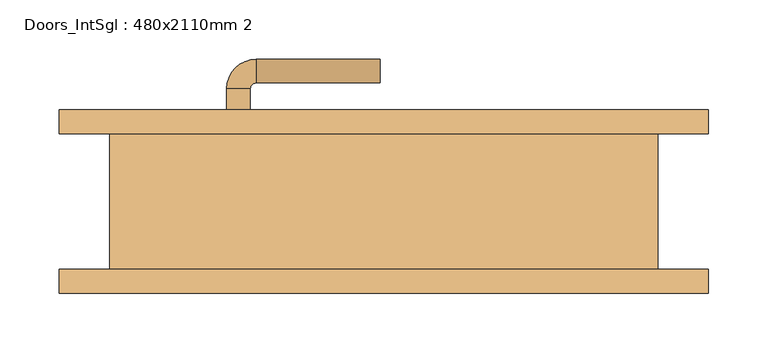
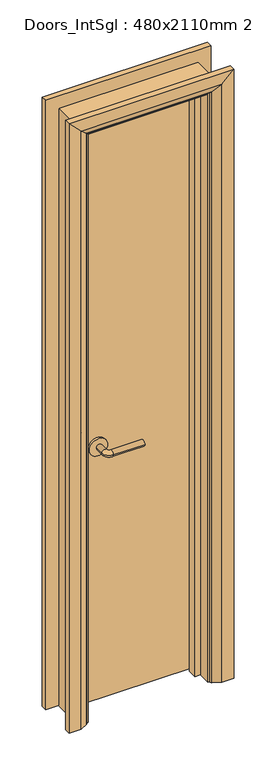
"""IFC4 building model written with IfcOpenShell, lengths in millimetres: door geometry, Doors_IntSgl : 480x2110mm 2."""

from ifc_helpers import new_model, si_unit, point, frame, frame_2d, origin, place, context, project, spatial, polyline, circle_curve, ellipse_curve, trimmed, segment, composite_curve, outline, extrude, faceted_brep, source, transform, mapped, element, save
from ifc_brep_helpers import plane_surface, cylinder_surface, revolved_surface, advanced_brep


def doors_intsgl_480x2110mm_2_fe7a8983(model_context):
    return source(origin(), model_context, "Body", "SolidModel", [
        advanced_brep(
        [(-133.0, 11.5, 900.0), (-113.0, 11.5, 900.0), (-113.0, -18.5, 900.0), (-133.0, -18.5, 900.0), (-108.0, -23.5, 900.0), (-108.0, -43.5, 900.0), (-3.0, -43.5, 900.0), (-3.0, -23.5, 900.0)],
        [
            (0, 1, circle_curve(frame((-123.0, 11.5, 900.0), z_axis=(0.0, 1.0, 0.0), x_axis=(1.0, 0.0, 0.0)), 10.0)),
            (1, 0, circle_curve(frame((-123.0, 11.5, 900.0), z_axis=(0.0, 1.0, 0.0), x_axis=(1.0, 0.0, 0.0)), 10.0)),
            (1, 2),
            (2, 3, circle_curve(frame((-123.0, -18.5, 900.0), z_axis=(0.0, 1.0, 0.0), x_axis=(1.0, 0.0, 0.0)), 10.0)),
            (3, 0),
            (3, 2, circle_curve(frame((-123.0, -18.5, 900.0), z_axis=(0.0, 1.0, 0.0), x_axis=(1.0, 0.0, 0.0)), 10.0)),
            (4, 5, circle_curve(frame((-108.0, -33.5, 900.0), z_axis=(-1.0, 0.0, 0.0), x_axis=(0.0, 1.0, 0.0)), 10.0)),
            (5, 3, circle_curve(frame((-108.0, -18.5, 900.0), z_axis=(0.0, 0.0, -1.0), x_axis=(-1.0, 0.0, 0.0)), 25.0)),
            (2, 4, circle_curve(frame((-108.0, -18.5, 900.0), z_axis=(0.0, 0.0, 1.0), x_axis=(-1.0, 0.0, 0.0)), 5.0)),
            (5, 4, circle_curve(frame((-108.0, -33.5, 900.0), z_axis=(-1.0, 0.0, 0.0), x_axis=(0.0, 1.0, 0.0)), 10.0)),
            (6, 7, circle_curve(frame((-3.0, -33.5, 900.0), z_axis=(1.0, 0.0, 0.0), x_axis=(0.0, 1.0, 0.0)), 10.0)),
            (7, 6, circle_curve(frame((-3.0, -33.5, 900.0), z_axis=(1.0, 0.0, 0.0), x_axis=(0.0, 1.0, 0.0)), 10.0)),
            (4, 7),
            (6, 5),
        ],
        [
            plane_surface(frame((-123.0, 11.5, 900.0), z_axis=(0.0, 1.0, 0.0), x_axis=(0.0, 0.0, 1.0))),
            cylinder_surface(frame((-123.0, 11.5, 900.0), z_axis=(0.0, 1.0, 0.0), x_axis=(1.0, 0.0, 0.0)), 10.0),
            revolved_surface(trimmed(ellipse_curve(frame((-123.0, -18.5, 900.0), z_axis=(0.0, -1.0, 0.0), x_axis=(1.0, 0.0, 0.0)), 10.0, 10.0), [point((-133.0, -18.5, 900.0))], [point((-113.0, -18.5, 900.0))], True, "CARTESIAN"), (-108.0, -18.5, 900.0), (0.0, 0.0, -1.0)),
            revolved_surface(trimmed(ellipse_curve(frame((-123.0, -18.5, 900.0), z_axis=(0.0, -1.0, 0.0), x_axis=(1.0, 0.0, 0.0)), 10.0, 10.0), [point((-113.0, -18.5, 900.0))], [point((-133.0, -18.5, 900.0))], True, "CARTESIAN"), (-108.0, -18.5, 900.0), (0.0, 0.0, -1.0)),
            plane_surface(frame((-3.0, -33.5, 900.0), z_axis=(1.0, 0.0, 0.0), x_axis=(0.0, 0.0, 1.0))),
            cylinder_surface(frame((-108.0, -33.5, 900.0), z_axis=(-1.0, 0.0, 0.0), x_axis=(0.0, 1.0, 0.0)), 10.0),
        ],
        [
            (0, [[1, 2]]),
            (1, [[3, 4, 5, -2]]),
            (1, [[-5, 6, -3, -1]]),
            (2, [[7, 8, -4, 9]]),
            (3, [[10, -9, -6, -8]]),
            (4, [[11, 12]]),
            (5, [[13, -11, 14, -7]]),
            (5, [[-14, -12, -13, -10]]),
        ],
    ),
        extrude(outline(composite_curve([segment(trimmed(circle_curve(frame_2d((900.0, -125.5)), 30.0), [point((900.0, -155.5))], [point((900.0, -95.5))], False, "CARTESIAN"), True, "CONTINUOUS"), segment(trimmed(circle_curve(frame_2d((900.0, -125.5)), 30.0), [point((900.0, -95.5))], [point((900.0, -155.5))], False, "CARTESIAN"), True, "CONTINUOUS")], self_intersect=False)), frame((0.0, 11.5, 0.0), z_axis=(0.0, 1.0, 0.0), x_axis=(0.0, 0.0, 1.0)), (0.0, 0.0, 1.0), 8.0),
        advanced_brep(
        [(-133.0, 65.5, 900.0), (-113.0, 65.5, 900.0), (-133.0, 95.5, 900.0), (-113.0, 95.5, 900.0), (-108.0, 100.5, 900.0), (-108.0, 120.5, 900.0), (-3.0, 120.5, 900.0), (-3.0, 100.5, 900.0)],
        [
            (0, 1, circle_curve(frame((-123.0, 65.5, 900.0), z_axis=(0.0, -1.0, 0.0), x_axis=(1.0, 0.0, 0.0)), 10.0)),
            (1, 0, circle_curve(frame((-123.0, 65.5, 900.0), z_axis=(0.0, -1.0, 0.0), x_axis=(1.0, 0.0, 0.0)), 10.0)),
            (0, 2),
            (2, 3, circle_curve(frame((-123.0, 95.5, 900.0), z_axis=(0.0, -1.0, 0.0), x_axis=(1.0, 0.0, 0.0)), 10.0)),
            (3, 1),
            (3, 2, circle_curve(frame((-123.0, 95.5, 900.0), z_axis=(0.0, -1.0, 0.0), x_axis=(1.0, 0.0, 0.0)), 10.0)),
            (4, 3, circle_curve(frame((-108.0, 95.5, 900.0), z_axis=(0.0, 0.0, 1.0), x_axis=(-1.0, 0.0, 0.0)), 5.0)),
            (2, 5, circle_curve(frame((-108.0, 95.5, 900.0), z_axis=(0.0, 0.0, -1.0), x_axis=(-1.0, 0.0, 0.0)), 25.0)),
            (5, 4, circle_curve(frame((-108.0, 110.5, 900.0), z_axis=(-1.0, 0.0, 0.0), x_axis=(0.0, -1.0, 0.0)), 10.0)),
            (4, 5, circle_curve(frame((-108.0, 110.5, 900.0), z_axis=(-1.0, 0.0, 0.0), x_axis=(0.0, -1.0, 0.0)), 10.0)),
            (6, 7, circle_curve(frame((-3.0, 110.5, 900.0), z_axis=(1.0, 0.0, 0.0), x_axis=(0.0, -1.0, 0.0)), 10.0)),
            (7, 6, circle_curve(frame((-3.0, 110.5, 900.0), z_axis=(1.0, 0.0, 0.0), x_axis=(0.0, -1.0, 0.0)), 10.0)),
            (5, 6),
            (7, 4),
        ],
        [
            plane_surface(frame((-123.0, 65.5, 900.0), z_axis=(0.0, -1.0, 0.0), x_axis=(0.0, 0.0, 1.0))),
            cylinder_surface(frame((-123.0, 65.5, 900.0), z_axis=(0.0, -1.0, 0.0), x_axis=(1.0, 0.0, 0.0)), 10.0),
            revolved_surface(trimmed(ellipse_curve(frame((-123.0, 95.5, 900.0), z_axis=(0.0, -1.0, 0.0), x_axis=(1.0, 0.0, 0.0)), 10.0, 10.0), [point((-133.0, 95.5, 900.0))], [point((-113.0, 95.5, 900.0))], True, "CARTESIAN"), (-108.0, 95.5, 900.0), (0.0, 0.0, -1.0)),
            revolved_surface(trimmed(ellipse_curve(frame((-123.0, 95.5, 900.0), z_axis=(0.0, -1.0, 0.0), x_axis=(1.0, 0.0, 0.0)), 10.0, 10.0), [point((-113.0, 95.5, 900.0))], [point((-133.0, 95.5, 900.0))], True, "CARTESIAN"), (-108.0, 95.5, 900.0), (0.0, 0.0, -1.0)),
            plane_surface(frame((-3.0, 110.5, 900.0), z_axis=(1.0, 0.0, 0.0), x_axis=(0.0, 0.0, 1.0))),
            cylinder_surface(frame((-108.0, 110.5, 900.0), z_axis=(-1.0, 0.0, 0.0), x_axis=(0.0, -1.0, 0.0)), 10.0),
        ],
        [
            (0, [[1, 2]]),
            (1, [[-1, 3, 4, 5]]),
            (1, [[-2, -5, 6, -3]]),
            (2, [[7, -4, 8, 9]]),
            (3, [[-8, -6, -7, 10]]),
            (4, [[11, 12]]),
            (5, [[-9, 13, -12, 14]]),
            (5, [[-10, -14, -11, -13]]),
        ],
    ),
        extrude(outline(composite_curve([segment(trimmed(circle_curve(frame_2d((900.0, -125.5)), 30.0), [point((900.0, -155.5))], [point((900.0, -95.5))], False, "CARTESIAN"), True, "CONTINUOUS"), segment(trimmed(circle_curve(frame_2d((900.0, -125.5)), 30.0), [point((900.0, -95.5))], [point((900.0, -155.5))], False, "CARTESIAN"), True, "CONTINUOUS")], self_intersect=False)), frame((0.0, 57.5, 0.0), z_axis=(0.0, 1.0, 0.0), x_axis=(0.0, 0.0, 1.0)), (0.0, 0.0, 1.0), 8.0),
        extrude(outline(polyline([(198.0, 19.5), (-198.0, 19.5), (-198.0, 57.5), (198.0, 57.5), (198.0, 19.5)])), frame((0.0, 0.0, 8.0), z_axis=(0.0, 0.0, 1.0), x_axis=(1.0, 0.0, 0.0)), (0.0, 0.0, 1.0), 2060.0),
        advanced_brep(
        [(275.0, 77.5, 0.0), (275.0, 57.5, 0.0), (205.0, 57.5, 0.0), (209.0, 63.5, 0.0), (235.0, 77.5, 0.0), (275.0, 77.5, 2145.0), (275.0, 57.5, 2145.0), (-275.0, 57.5, 2145.0), (-275.0, 57.5, 0.0), (-205.0, 57.5, 0.0), (-205.0, 57.5, 2075.0), (205.0, 57.5, 2075.0), (209.0, 63.5, 2079.0), (235.0, 77.5, 2105.0), (-235.0, 77.5, 2105.0), (-235.0, 77.5, 0.0), (-275.0, 77.5, 0.0), (-275.0, 77.5, 2145.0), (-209.0, 63.5, 0.0), (-209.0, 63.5, 2079.0)],
        [
            (0, 1),
            (1, 2),
            (2, 3, circle_curve(frame((213.0, 56.5, 0.0), z_axis=(0.0, 0.0, -1.0), x_axis=(1.0, 0.0, 0.0)), 8.0622577)),
            (3, 4),
            (4, 0),
            (0, 5),
            (5, 6),
            (6, 1),
            (6, 7),
            (7, 8),
            (8, 9),
            (9, 10),
            (10, 11),
            (11, 2),
            (11, 12, ellipse_curve(frame((213.0, 56.5, 2083.0), z_axis=(0.7071067811865475, 0.0, -0.7071067811865475), x_axis=(-0.7071067811865474, 0.0, -0.7071067811865476)), 11.4017543, 8.0622577)),
            (12, 3),
            (12, 13),
            (13, 4),
            (13, 14),
            (14, 15),
            (15, 16),
            (16, 17),
            (17, 5),
            (7, 17),
            (16, 8),
            (15, 18),
            (18, 9, circle_curve(frame((-213.0, 56.5, 0.0), z_axis=(0.0, 0.0, -1.0), x_axis=(-1.0, 0.0, 0.0)), 8.0622577)),
            (19, 10, ellipse_curve(frame((-213.0, 56.5, 2083.0), z_axis=(-0.7071067811865475, 0.0, -0.7071067811865475), x_axis=(-0.7071067811865474, 0.0, 0.7071067811865476)), 11.4017543, 8.0622577)),
            (18, 19),
            (14, 19),
            (19, 12),
        ],
        [
            plane_surface(frame((205.0, 57.5, 0.0), z_axis=(0.0, 0.0, -1.0), x_axis=(0.0, -1.0, 0.0))),
            plane_surface(frame((275.0, 77.5, 0.0), z_axis=(1.0, 0.0, 0.0), x_axis=(0.0, 0.0, 1.0))),
            plane_surface(frame((275.0, 57.5, 0.0), z_axis=(0.0, -1.0, 0.0), x_axis=(0.0, 0.0, 1.0))),
            cylinder_surface(frame((213.0, 56.5, 0.0), z_axis=(0.0, 0.0, -1.0), x_axis=(1.0, 0.0, 0.0)), 8.0622577),
            plane_surface(frame((209.0, 63.5, 0.0), z_axis=(-0.4740998230350126, 0.880471099922178, 0.0), x_axis=(0.0, 0.0, 1.0))),
            plane_surface(frame((235.0, 77.5, 0.0), z_axis=(0.0, 1.0, 0.0), x_axis=(0.0, 0.0, 1.0))),
            plane_surface(frame((-275.0, 77.5, 2145.0), z_axis=(-1.0, 0.0, 0.0), x_axis=(0.0, 0.0, -1.0))),
            plane_surface(frame((-205.0, 57.5, 0.0), z_axis=(0.0, 0.0, -1.0), x_axis=(0.0, -1.0, 0.0))),
            cylinder_surface(frame((-213.0, 56.5, 2075.0), z_axis=(0.0, 0.0, 1.0), x_axis=(-1.0, 0.0, 0.0)), 8.0622577),
            plane_surface(frame((-209.0, 63.5, 2079.0), z_axis=(0.47409982303501824, 0.8804710999221749, 0.0), x_axis=(0.0, 0.0, -1.0))),
            plane_surface(frame((275.0, 77.5, 2145.0), z_axis=(0.0, 0.0, 1.0), x_axis=(-1.0, 0.0, 0.0))),
            cylinder_surface(frame((205.0, 56.5, 2083.0), z_axis=(1.0, 0.0, 0.0), x_axis=(0.0, 0.0, 1.0)), 8.0622577),
            plane_surface(frame((209.0, 63.5, 2079.0), z_axis=(0.0, 0.8804710999221764, -0.4740998230350154), x_axis=(-1.0, 0.0, 0.0))),
        ],
        [
            (0, [[1, 2, 3, 4, 5]]),
            (1, [[-1, 6, 7, 8]]),
            (2, [[-2, -8, 9, 10, 11, 12, 13, 14]]),
            (3, [[-3, -14, 15, 16]]),
            (4, [[-4, -16, 17, 18]]),
            (5, [[-5, -18, 19, 20, 21, 22, 23, -6]]),
            (6, [[24, -22, 25, -10]]),
            (7, [[-21, 26, 27, -11, -25]]),
            (8, [[28, -12, -27, 29]]),
            (9, [[30, -29, -26, -20]]),
            (10, [[-7, -23, -24, -9]]),
            (11, [[-15, -13, -28, 31]]),
            (12, [[-17, -31, -30, -19]]),
        ],
    ),
        extrude(outline(polyline([(0.0, -200.0), (0.0, -181.0), (2051.0, -181.0), (2051.0, 181.0), (0.0, 181.0), (0.0, 200.0), (2070.0, 200.0), (2070.0, -200.0), (0.0, -200.0)])), frame((0.0, -14.5, 0.0), z_axis=(0.0, 1.0, 0.0), x_axis=(0.0, 0.0, 1.0)), (0.0, 0.0, 1.0), 32.0),
        advanced_brep(
        [(-275.0, -77.5, 0.0), (-275.0, -57.5, 0.0), (-205.0, -57.5, 0.0), (-209.0, -63.5, 0.0), (-235.0, -77.5, 0.0), (-275.0, -77.5, 2145.0), (-275.0, -57.5, 2145.0), (-205.0, -57.5, 2075.0), (-209.0, -63.5, 2079.0), (-235.0, -77.5, 2105.0), (275.0, -77.5, 0.0), (235.0, -77.5, 0.0), (209.0, -63.5, 0.0), (205.0, -57.5, 0.0), (275.0, -57.5, 0.0), (275.0, -77.5, 2145.0), (235.0, -77.5, 2105.0), (209.0, -63.5, 2079.0), (205.0, -57.5, 2075.0), (275.0, -57.5, 2145.0)],
        [
            (0, 1),
            (1, 2),
            (2, 3, circle_curve(frame((-213.0, -56.5, 0.0), z_axis=(0.0, 0.0, -1.0), x_axis=(-1.0, 0.0, 0.0)), 8.0622577)),
            (3, 4),
            (4, 0),
            (0, 5),
            (5, 6),
            (6, 1),
            (6, 7),
            (7, 2),
            (7, 8, ellipse_curve(frame((-213.0, -56.5, 2083.0), z_axis=(-0.7071067811865475, 0.0, -0.7071067811865475), x_axis=(0.7071067811865474, 0.0, -0.7071067811865476)), 11.4017543, 8.0622577)),
            (8, 3),
            (8, 9),
            (9, 4),
            (9, 5),
            (10, 11),
            (11, 12),
            (12, 13, circle_curve(frame((213.0, -56.5, 0.0), z_axis=(0.0, 0.0, -1.0), x_axis=(1.0, 0.0, 0.0)), 8.0622577)),
            (13, 14),
            (14, 10),
            (15, 16),
            (16, 11),
            (10, 15),
            (16, 17),
            (17, 12),
            (17, 18, ellipse_curve(frame((213.0, -56.5, 2083.0), z_axis=(0.7071067811865475, 0.0, -0.7071067811865475), x_axis=(0.7071067811865474, 0.0, 0.7071067811865476)), 11.4017543, 8.0622577)),
            (18, 13),
            (18, 19),
            (19, 14),
            (19, 15),
            (5, 15),
            (19, 6),
            (18, 7),
            (17, 8),
            (16, 9),
        ],
        [
            plane_surface(frame((-205.0, -130.3010989, 0.0), z_axis=(0.0, 0.0, -1.0), x_axis=(1.0, 0.0, 0.0))),
            plane_surface(frame((-275.0, -77.5, 0.0), z_axis=(-1.0, 0.0, 0.0), x_axis=(0.0, 0.0, 1.0))),
            plane_surface(frame((-275.0, -57.5, 0.0), z_axis=(0.0, 1.0, 0.0), x_axis=(0.0, 0.0, 1.0))),
            cylinder_surface(frame((-213.0, -56.5, 0.0), z_axis=(0.0, 0.0, -1.0), x_axis=(-1.0, 0.0, 0.0)), 8.0622577),
            plane_surface(frame((-209.0, -63.5, 0.0), z_axis=(0.4740998230350183, -0.8804710999221749, 0.0), x_axis=(0.0, 0.0, 1.0))),
            plane_surface(frame((-235.0, -77.5, 0.0), z_axis=(0.0, -1.0, 0.0), x_axis=(0.0, 0.0, 1.0))),
            plane_surface(frame((205.0, -130.3010989, 0.0), z_axis=(0.0, 0.0, -1.0), x_axis=(-1.0, 0.0, 0.0))),
            plane_surface(frame((235.0, -77.5, 2105.0), z_axis=(0.0, -1.0, 0.0), x_axis=(0.0, 0.0, -1.0))),
            plane_surface(frame((209.0, -63.5, 2079.0), z_axis=(-0.4740998230350183, -0.8804710999221749, 0.0), x_axis=(0.0, 0.0, -1.0))),
            cylinder_surface(frame((213.0, -56.5, 2075.0), z_axis=(0.0, 0.0, 1.0), x_axis=(1.0, 0.0, 0.0)), 8.0622577),
            plane_surface(frame((275.0, -57.5, 2145.0), z_axis=(0.0, 1.0, 0.0), x_axis=(0.0, 0.0, -1.0))),
            plane_surface(frame((275.0, -77.5, 2145.0), z_axis=(1.0, 0.0, 0.0), x_axis=(0.0, 0.0, -1.0))),
            plane_surface(frame((-275.0, -77.5, 2145.0), z_axis=(0.0, 0.0, 1.0), x_axis=(1.0, 0.0, 0.0))),
            plane_surface(frame((-275.0, -57.5, 2145.0), z_axis=(0.0, 1.0, 0.0), x_axis=(1.0, 0.0, 0.0))),
            cylinder_surface(frame((-205.0, -56.5, 2083.0), z_axis=(-1.0, 0.0, 0.0), x_axis=(0.0, 0.0, 1.0)), 8.0622577),
            plane_surface(frame((-209.0, -63.5, 2079.0), z_axis=(0.0, -0.8804710999221749, -0.4740998230350183), x_axis=(1.0, 0.0, 0.0))),
            plane_surface(frame((-235.0, -77.5, 2105.0), z_axis=(0.0, -1.0, 0.0), x_axis=(1.0, 0.0, 0.0))),
        ],
        [
            (0, [[1, 2, 3, 4, 5]]),
            (1, [[-1, 6, 7, 8]]),
            (2, [[-2, -8, 9, 10]]),
            (3, [[-3, -10, 11, 12]]),
            (4, [[-4, -12, 13, 14]]),
            (5, [[-5, -14, 15, -6]]),
            (6, [[16, 17, 18, 19, 20]]),
            (7, [[21, 22, -16, 23]]),
            (8, [[24, 25, -17, -22]]),
            (9, [[26, 27, -18, -25]]),
            (10, [[28, 29, -19, -27]]),
            (11, [[30, -23, -20, -29]]),
            (12, [[-7, 31, -30, 32]]),
            (13, [[-9, -32, -28, 33]]),
            (14, [[-11, -33, -26, 34]]),
            (15, [[-13, -34, -24, 35]]),
            (16, [[-15, -35, -21, -31]]),
        ],
    ),
        faceted_brep([(-200.0, 57.5, 0.0), (-200.0, -57.5, 0.0), (-232.0, -57.5, 0.0), (-232.0, 57.5, 0.0), (-200.0, 57.5, 2070.0), (-200.0, -57.5, 2070.0), (-232.0, -57.5, 2102.0), (-232.0, 57.5, 2102.0), (200.0, 57.5, 0.0), (232.0, 57.5, 0.0), (232.0, -57.5, 0.0), (200.0, -57.5, 0.0), (200.0, 57.5, 2070.0), (232.0, 57.5, 2102.0), (232.0, -57.5, 2102.0), (200.0, -57.5, 2070.0)], [[[0, 1, 2, 3]], [[1, 0, 4, 5]], [[2, 1, 5, 6]], [[3, 2, 6, 7]], [[0, 3, 7, 4]], [[8, 9, 10, 11]], [[12, 13, 9, 8]], [[13, 14, 10, 9]], [[14, 15, 11, 10]], [[15, 12, 8, 11]], [[5, 4, 12, 15]], [[6, 5, 15, 14]], [[7, 6, 14, 13]], [[4, 7, 13, 12]]]),
    ])


if __name__ == "__main__":
    model = new_model("IFC4")
    model_context = context("Model", 3, world=origin())
    ifc_project = project(units=[si_unit("LENGTHUNIT", "METRE", prefix="MILLI")], contexts=[model_context])
    site = spatial("IfcSite", under=ifc_project)
    building = spatial("IfcBuilding", under=site)
    placement = place(None, origin())
    doors_intsgl_480x2110mm_2_shape = doors_intsgl_480x2110mm_2_fe7a8983(model_context)
    element("IfcDoor", 1, ObjectType="Doors_IntSgl : 480x2110mm 2", at=placement, inside=building, context=model_context, shape_type="MappedRepresentation", body=[
        mapped(doors_intsgl_480x2110mm_2_shape, transform((0.0, 0.0, 0.0), x_axis=(1.0, 0.0, 0.0), y_axis=(0.0, 1.0, 0.0), z_axis=(0.0, 0.0, 1.0))),
    ])
    save(model, "model.ifc")

# Revit data of these elements
# Type "Doors_IntSgl : 480x2110mm 2"
#   Type Mark = "47"
#   Type Comments = "Internal Single"
#   Operation = "SingleSwingRight"
#   Manufacturer = "Revit"
#   Keynote = "L20"
#   Description = "Internal Single Door"
#   Analytic Construction = "Metal"
#   UnderCut = 8 mm
#   Tolerance = 2 mm
#   Thickness = 38 mm
#   Thermal Resistance (R) = 0.270117 (m²·K)/W
#   Structural Tolerance = 8 mm
#   StopDepth = 32 mm
#   Stop Thickness = 19 mm
#   Rough Width = 480 mm
#   Rough Height = 2110 mm
#   Height to Top Lock Rail = 1000 mm
#   Heat Transfer Coefficient (U) = 3.7021 W/(m²·K)
#   Handle Z Distance = 900 mm
#   Handle X Distance = 75 mm
#   Frame Thickness = 32 mm
#   Door Panel Width = 396 mm
#   Door Panel Thickness = 38 mm
#   Door Panel Offset = 0 mm
#   Height = 2110 mm
#   Width = 480 mm
#   Door Panel Height = 2060 mm
#   Architrave Setback = 5 mm
#   Vis - Ironmongery = yes
#   Material Ironmongery = Door - Handle
#   Material Frame = Door - Frame/Mullion (1)
#   Material Door = Door - Panel
#   Material Architrave = Door - Architrave
#   Visual Light Transmittance = 0
#   Solar Heat Gain Coefficient = 0
#   Function = (empty or 0)
#   Wall Closure = (empty or 0)
# Element 1 (IfcDoor, "Doors_IntSgl : 480x2110mm 2")
#   Materials on its faces: "Door - Architrave", "Door - Handle", "Door - Frame/Mullion (1)", "Door - Panel"
# Materials
#   "Door - Handle": class "Miscellaneous", colour RGB 0 0 0, transparency 0, Keynote = "P21", Cost = 0
#   "Door - Frame/Mullion (1)": class "Wood", colour RGB 212 179 113, transparency 0, Keynote = "L20", Cost = 0
#   "Door - Panel": class "Wood", colour RGB 210 159 95, transparency 0, Keynote = "L20", Cost = 0
#   "Door - Architrave": class "Wood", colour RGB 154 90 5, transparency 0, Keynote = "P20", Cost = 0
